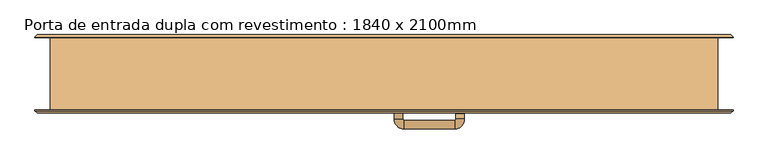
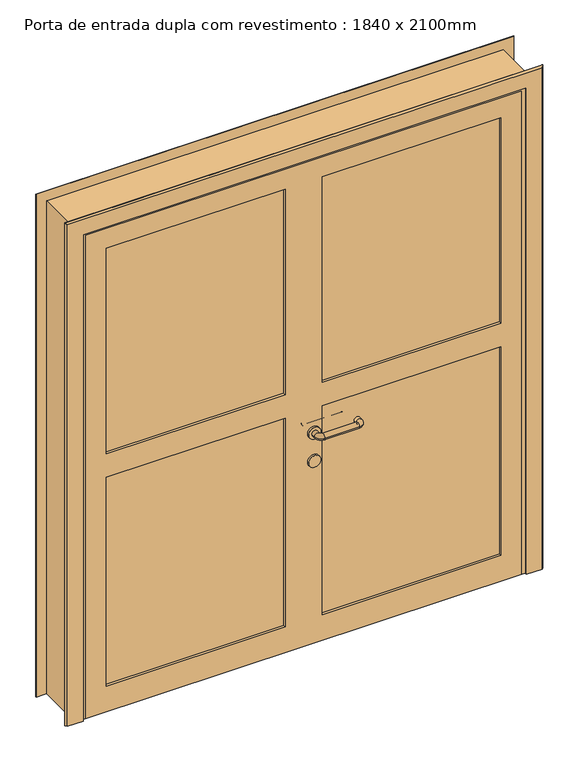
"""IFC4 building model written with IfcOpenShell, lengths in millimetres: door geometry, Porta de entrada dupla com revestimento : 1840 x 2100mm."""

import ifcopenshell
import ifcopenshell.guid

model = None  # the IFC model being written
_history = None  # IfcOwnerHistory: only IFC2X3 demands one
_inside = {}  # id of a spatial element -> (the spatial element, [elements in it])
_under = {}  # id of a project, library or spatial element -> (it, [spatial elements below it])
_declared = {}  # id of a project -> (the project, [libraries it declares])
_typed = {}  # id of a type object -> (the type object, [elements of that type])
_made_of = {}  # id of a material, layer set ... -> (it, [elements and type objects made of it])


def new_model(schema):
    """Start an empty IFC model of exactly this schema.

    Asked for "IFC4X3", IfcOpenShell would pick the latest addendum, in which some entities
    have other attributes; the version numbers below select the first issue.
    IFC2X3 requires an IfcOwnerHistory on every rooted entity: one is made here for all.
    """
    global model, _history
    if schema == "IFC4X3":
        model = ifcopenshell.file(schema_version=(4, 3, 0, 0))
    else:
        model = ifcopenshell.file(schema=schema)
    _inside.clear()
    _under.clear()
    _declared.clear()
    _typed.clear()
    _made_of.clear()
    _history = None
    if model.schema == "IFC2X3":
        org = make("IfcOrganization", Name="unknown")
        user = make(
            "IfcPersonAndOrganization",
            ThePerson=make("IfcPerson", FamilyName="unknown"),
            TheOrganization=org,
        )
        app = make(
            "IfcApplication",
            ApplicationDeveloper=org,
            Version="unknown",
            ApplicationFullName="unknown",
            ApplicationIdentifier="unknown",
        )
        _history = make(
            "IfcOwnerHistory",
            OwningUser=user,
            OwningApplication=app,
            ChangeAction="ADDED",
            CreationDate=0,
        )
    return model


def make(cls, **values):
    """One entity of the class cls with the attributes given. An attribute that is None is left unset."""
    return model.create_entity(
        cls, **{name: value for name, value in values.items() if value is not None}
    )


def rooted(cls, **values):
    """An entity with a GlobalId (a new one), such as an element, a storey or a relation."""
    return make(cls, GlobalId=ifcopenshell.guid.new(), OwnerHistory=_history, **values)


def si_unit(unit_type, name, prefix=None):
    """IfcSIUnit, for example si_unit("LENGTHUNIT", "METRE", prefix="MILLI")."""
    return make("IfcSIUnit", UnitType=unit_type, Prefix=prefix, Name=name)


def assignment(units):
    """IfcUnitAssignment: the units of a project."""
    return None if units is None else make("IfcUnitAssignment", Units=units)


def point(xyz):
    """IfcCartesianPoint."""
    return None if xyz is None else make("IfcCartesianPoint", Coordinates=xyz)


def direction(xyz):
    """IfcDirection."""
    return None if xyz is None else make("IfcDirection", DirectionRatios=xyz)


def frame(location, z_axis=None, x_axis=None):
    """IfcAxis2Placement3D, a coordinate frame: its origin and axes. An axis left out is left unset."""
    return make(
        "IfcAxis2Placement3D",
        Location=point(location),
        Axis=direction(z_axis),
        RefDirection=direction(x_axis),
    )


def frame_2d(location, x_axis=None):
    """IfcAxis2Placement2D, a coordinate frame in the plane: its origin and x axis."""
    return make(
        "IfcAxis2Placement2D", Location=point(location), RefDirection=direction(x_axis)
    )


def origin():
    """The frame at (0, 0, 0) with its axes left unset."""
    return frame((0.0, 0.0, 0.0))


def place(relative_to, where):
    """IfcLocalPlacement: puts the frame where relative to a parent placement (None: the world)."""
    return make(
        "IfcLocalPlacement", PlacementRelTo=relative_to, RelativePlacement=where
    )


def context(
    kind, dimensions, precision=None, world=None, true_north=None, identifier=None
):
    """IfcGeometricRepresentationContext, for example the 3D "Model" context."""
    return make(
        "IfcGeometricRepresentationContext",
        ContextIdentifier=identifier,
        ContextType=kind,
        CoordinateSpaceDimension=dimensions,
        Precision=precision,
        WorldCoordinateSystem=world,
        TrueNorth=true_north,
    )


def project(units=None, contexts=None):
    """IfcProject with its units and contexts."""
    return rooted(
        "IfcProject",
        Name="project",
        RepresentationContexts=contexts,
        UnitsInContext=assignment(units),
    )


def spatial(cls, under=None, at=None, **own):
    """A site, building, storey or space (cls), placed at a placement, below another one or the project."""
    s = rooted(cls, ObjectPlacement=at, **own)
    if under is not None:
        _under.setdefault(under.id(), (under, []))[1].append(s)
    return s


def polyline(points):
    """IfcPolyline through the points."""
    return make("IfcPolyline", Points=[point(p) for p in points])


def circle_curve(where, radius):
    """IfcCircle in the frame where."""
    return make("IfcCircle", Position=where, Radius=radius)


def ellipse_curve(where, semi_axis1, semi_axis2):
    """IfcEllipse in the frame where."""
    return make(
        "IfcEllipse", Position=where, SemiAxis1=semi_axis1, SemiAxis2=semi_axis2
    )


def trimmed(basis, trim1, trim2, sense, master):
    """IfcTrimmedCurve: the piece of a basis curve between two trims."""
    return make(
        "IfcTrimmedCurve",
        BasisCurve=basis,
        Trim1=trim1,
        Trim2=trim2,
        SenseAgreement=sense,
        MasterRepresentation=master,
    )


def segment(curve, same_sense, transition):
    """IfcCompositeCurveSegment."""
    return make(
        "IfcCompositeCurveSegment",
        Transition=transition,
        SameSense=same_sense,
        ParentCurve=curve,
    )


def composite_curve(segments, self_intersect=None):
    """IfcCompositeCurve: segments joined end to end."""
    return make("IfcCompositeCurve", Segments=segments, SelfIntersect=self_intersect)


def outline(outer, holes=None, kind="AREA"):
    """IfcArbitraryClosedProfileDef: a profile drawn as a closed curve; with holes, ...WithVoids."""
    if holes is None:
        return make("IfcArbitraryClosedProfileDef", ProfileType=kind, OuterCurve=outer)
    return make(
        "IfcArbitraryProfileDefWithVoids",
        ProfileType=kind,
        OuterCurve=outer,
        InnerCurves=holes,
    )


def extrude(swept, where, along, depth):
    """IfcExtrudedAreaSolid: the profile swept, set in the frame where, extruded along a direction by depth."""
    return make(
        "IfcExtrudedAreaSolid",
        SweptArea=swept,
        Position=where,
        ExtrudedDirection=direction(along),
        Depth=depth,
    )


def faces_of(points, faces, orient=None, outer=None):
    """IfcFace entities. A face is a list of loops; a loop is a list of indices into points, from 0.

    orient and outer hold one flag for each loop. By default every Orientation is true, the
    first loop of a face is its IfcFaceOuterBound and the others are IfcFaceBound.
    """
    made = []
    for i, loops in enumerate(faces):
        bounds = []
        for j, loop in enumerate(loops):
            is_outer = j == 0 if outer is None else outer[i][j]
            bounds.append(
                make(
                    "IfcFaceOuterBound" if is_outer else "IfcFaceBound",
                    Bound=make("IfcPolyLoop", Polygon=[points[k] for k in loop]),
                    Orientation=True if orient is None else orient[i][j],
                )
            )
        made.append(make("IfcFace", Bounds=bounds))
    return made


def faceted_brep(points, faces, orient=None, outer=None, voids=None):
    """IfcFacetedBrep: a solid bounded by flat faces; with voids (closed shells), ...WithVoids."""
    shared = [point(p) for p in points]
    hull = make("IfcClosedShell", CfsFaces=faces_of(shared, faces, orient, outer))
    if voids is None:
        return make("IfcFacetedBrep", Outer=hull)
    return make(
        "IfcFacetedBrepWithVoids",
        Outer=hull,
        Voids=[
            make(cls, CfsFaces=faces_of(shared, fs, o, b)) for cls, fs, o, b in voids
        ],
    )


def shape(context_of_items, identifier, shape_type, items):
    """IfcShapeRepresentation: the items that make up one representation, for example the "Body"."""
    return make(
        "IfcShapeRepresentation",
        ContextOfItems=context_of_items,
        RepresentationIdentifier=identifier,
        RepresentationType=shape_type,
        Items=items,
    )


def source(mapping_origin, context_of_items, identifier, shape_type, items):
    """IfcRepresentationMap: a shape defined once, which mapped items show again and again."""
    return make(
        "IfcRepresentationMap",
        MappingOrigin=mapping_origin,
        MappedRepresentation=shape(context_of_items, identifier, shape_type, items),
    )


def transform(
    local_origin,
    x_axis=None,
    y_axis=None,
    z_axis=None,
    scale=None,
    scale2=None,
    scale3=None,
    uniform=True,
):
    """IfcCartesianTransformationOperator3D, or its non-uniform kind. x_axis, y_axis, z_axis: its Axis1, 2, 3."""
    if uniform:
        return make(
            "IfcCartesianTransformationOperator3D",
            Axis1=direction(x_axis),
            Axis2=direction(y_axis),
            LocalOrigin=point(local_origin),
            Scale=scale,
            Axis3=direction(z_axis),
        )
    return make(
        "IfcCartesianTransformationOperator3DnonUniform",
        Axis1=direction(x_axis),
        Axis2=direction(y_axis),
        LocalOrigin=point(local_origin),
        Scale=scale,
        Axis3=direction(z_axis),
        Scale2=scale2,
        Scale3=scale3,
    )


def mapped(mapping_source, mapping_target):
    """IfcMappedItem: shows the shape of a source again, moved by a transform."""
    return make(
        "IfcMappedItem", MappingSource=mapping_source, MappingTarget=mapping_target
    )


def made_of(thing, what):
    """Note that an element or type object is made of a material, layer set ...; save() writes the relation."""
    if what is not None:
        _made_of.setdefault(what.id(), (what, []))[1].append(thing)
    return thing


def element(
    cls,
    number,
    at=None,
    inside=None,
    cuts=None,
    type_object=None,
    material=None,
    context=None,
    identifier="Body",
    shape_type=None,
    held_by="IfcProductDefinitionShape",
    body=None,
    shapes=None,
    **own,
):
    """One element of the class cls, such as IfcWall. Its Tag is "e" and its number.

    at: its placement. inside: the storey or other place that contains it. cuts: it is an
    opening in that element (IfcRelVoidsElement). A single representation is given by context,
    identifier, shape_type and body (its items); several are given by shapes. held_by: the class
    of the entity that holds the representations. save() writes the other relations.
    """
    e = rooted(cls, Tag="e%d" % number, ObjectPlacement=at, **own)
    if body is not None:
        shapes = [shape(context, identifier, shape_type, body)]
    if shapes is not None:
        e.Representation = make(held_by, Representations=shapes)
    if inside is not None:
        _inside.setdefault(inside.id(), (inside, []))[1].append(e)
    if cuts is not None:
        rooted(
            "IfcRelVoidsElement", RelatingBuildingElement=cuts, RelatedOpeningElement=e
        )
    if type_object is not None:
        _typed.setdefault(type_object.id(), (type_object, []))[1].append(e)
    return made_of(e, material)


def aggregate(whole, parts):
    """IfcRelAggregates: a whole, such as a stair, and the parts it consists of."""
    return rooted("IfcRelAggregates", RelatingObject=whole, RelatedObjects=parts)


def save(model, path):
    """Write the relations noted so far, then the file.

    IfcRelAggregates (storeys below a building ...), IfcRelContainedInSpatialStructure (elements
    in a storey), IfcRelDefinesByType, IfcRelAssociatesMaterial and IfcRelDeclares: one each for
    every whole, place, type object, material and project.
    """
    for whole, parts in _under.values():
        aggregate(whole, parts)
    for where, things in _inside.values():
        rooted(
            "IfcRelContainedInSpatialStructure",
            RelatedElements=things,
            RelatingStructure=where,
        )
    for kind, things in _typed.values():
        rooted("IfcRelDefinesByType", RelatedObjects=things, RelatingType=kind)
    for what, things in _made_of.values():
        rooted("IfcRelAssociatesMaterial", RelatedObjects=things, RelatingMaterial=what)
    for by, libraries in _declared.values():
        rooted("IfcRelDeclares", RelatingContext=by, RelatedDefinitions=libraries)
    model.write(path)


def plane_surface(at):
    """IfcPlane: the flat surface through the origin of the frame at, square to its z axis."""
    return make("IfcPlane", Position=at)


def cylinder_surface(at, radius):
    """IfcCylindricalSurface: all points at the distance radius from the z axis of the frame at."""
    return make("IfcCylindricalSurface", Position=at, Radius=radius)


def revolved_surface(curve, axis_point, axis_direction):
    """IfcSurfaceOfRevolution: the curve turned about the line through axis_point along axis_direction."""
    return make(
        "IfcSurfaceOfRevolution",
        SweptCurve=make("IfcArbitraryOpenProfileDef", ProfileType="CURVE", Curve=curve),
        AxisPosition=make("IfcAxis1Placement", Location=point(axis_point), Axis=direction(axis_direction)),
    )


def advanced_brep(points, edges, surfaces, faces):
    """IfcAdvancedBrep: a solid bounded by faces that lie on surfaces and meet in shared edges.

    An edge is (start, end): straight between two places in points (the first is 0);
    or (start, end, curve); or (start, end, curve, False) where it runs against its curve.
    A face is (place in surfaces, loops), or (place, loops, False) where it looks against
    its surface's normal. A loop lists edges by number (the first is 1), with a minus sign
    where the edge is run from its end to its start. The first loop is the outer one.
    """
    corners = [point(p) for p in points]
    vertices = [make("IfcVertexPoint", VertexGeometry=c) for c in corners]
    made = []
    for start, end, *more in edges:
        made.append(
            make(
                "IfcEdgeCurve",
                EdgeStart=vertices[start],
                EdgeEnd=vertices[end],
                EdgeGeometry=more[0] if more else make("IfcPolyline", Points=[corners[start], corners[end]]),
                SameSense=more[1] if len(more) > 1 else True,
            )
        )
    hull = []
    for where, loops, *sense in faces:
        bounds = []
        for j, loop in enumerate(loops):
            ring = [make("IfcOrientedEdge", EdgeElement=made[abs(k) - 1], Orientation=k > 0) for k in loop]
            bounds.append(
                make(
                    "IfcFaceOuterBound" if j == 0 else "IfcFaceBound",
                    Bound=make("IfcEdgeLoop", EdgeList=ring),
                    Orientation=True,
                )
            )
        hull.append(make("IfcAdvancedFace", Bounds=bounds, FaceSurface=surfaces[where], SameSense=sense[0] if sense else True))
    return make("IfcAdvancedBrep", Outer=make("IfcClosedShell", CfsFaces=hull))


def porta_de_entrada_dupla_com_revestimento_1840_x_2100mm_8bed4eb5(model_context):
    return source(origin(), model_context, "Body", "SolidModel", [
        advanced_brep(
        [(52.0, -57.0, 900.0), (28.0, -57.0, 900.0), (52.0, -40.0, 900.0), (28.0, -40.0, 900.0), (55.0, -13.0, 900.0), (55.0, -37.0, 900.0), (195.0, -37.0, 900.0), (195.0, -13.0, 900.0), (222.0, -40.0, 900.0), (198.0, -40.0, 900.0), (198.0, -55.0, 900.0), (222.0, -55.0, 900.0)],
        [
            (0, 1, circle_curve(frame((40.0, -57.0, 900.0), z_axis=(0.0, -1.0, 0.0), x_axis=(-1.0, 0.0, 0.0)), 12.0)),
            (1, 0, circle_curve(frame((40.0, -57.0, 900.0), z_axis=(0.0, -1.0, 0.0), x_axis=(-1.0, 0.0, 0.0)), 12.0)),
            (0, 2),
            (2, 3, circle_curve(frame((40.0, -40.0, 900.0), z_axis=(0.0, -1.0, 0.0), x_axis=(-1.0, 0.0, 0.0)), 12.0)),
            (3, 1),
            (3, 2, circle_curve(frame((40.0, -40.0, 900.0), z_axis=(0.0, -1.0, 0.0), x_axis=(-1.0, 0.0, 0.0)), 12.0)),
            (4, 3, circle_curve(frame((55.0, -40.0, 900.0), z_axis=(0.0, 0.0, 1.0), x_axis=(-1.0, 0.0, 0.0)), 27.0)),
            (2, 5, circle_curve(frame((55.0, -40.0, 900.0), z_axis=(0.0, 0.0, -1.0), x_axis=(-1.0, 0.0, 0.0)), 3.0)),
            (5, 4, circle_curve(frame((55.0, -25.0, 900.0), z_axis=(-1.0, 0.0, 0.0), x_axis=(0.0, 1.0, 0.0)), 12.0)),
            (4, 5, circle_curve(frame((55.0, -25.0, 900.0), z_axis=(-1.0, 0.0, 0.0), x_axis=(0.0, 1.0, 0.0)), 12.0)),
            (5, 6),
            (6, 7, circle_curve(frame((195.0, -25.0, 900.0), z_axis=(-1.0, 0.0, 0.0), x_axis=(0.0, 1.0, 0.0)), 12.0)),
            (7, 4),
            (7, 6, circle_curve(frame((195.0, -25.0, 900.0), z_axis=(-1.0, 0.0, 0.0), x_axis=(0.0, 1.0, 0.0)), 12.0)),
            (8, 7, circle_curve(frame((195.0, -40.0, 900.0), z_axis=(0.0, 0.0, 1.0), x_axis=(0.0, 1.0, 0.0)), 27.0)),
            (6, 9, circle_curve(frame((195.0, -40.0, 900.0), z_axis=(0.0, 0.0, -1.0), x_axis=(0.0, 1.0, 0.0)), 3.0)),
            (9, 8, circle_curve(frame((210.0, -40.0, 900.0), z_axis=(0.0, 1.0, 0.0), x_axis=(1.0, 0.0, 0.0)), 12.0)),
            (8, 9, circle_curve(frame((210.0, -40.0, 900.0), z_axis=(0.0, 1.0, 0.0), x_axis=(1.0, 0.0, 0.0)), 12.0)),
            (10, 11, circle_curve(frame((210.0, -55.0, 900.0), z_axis=(0.0, -1.0, 0.0), x_axis=(1.0, 0.0, 0.0)), 12.0)),
            (11, 10, circle_curve(frame((210.0, -55.0, 900.0), z_axis=(0.0, -1.0, 0.0), x_axis=(1.0, 0.0, 0.0)), 12.0)),
            (9, 10),
            (11, 8),
        ],
        [
            plane_surface(frame((-802.0, -57.0, 1730.0), z_axis=(0.0, -1.0, 0.0), x_axis=(0.0, 0.0, 1.0))),
            cylinder_surface(frame((40.0, -57.0, 900.0), z_axis=(0.0, -1.0, 0.0), x_axis=(-1.0, 0.0, 0.0)), 12.0),
            revolved_surface(trimmed(ellipse_curve(frame((40.0, -40.0, 900.0), z_axis=(0.0, -1.0, 0.0), x_axis=(-1.0, 0.0, 0.0)), 12.0, 12.0), [point((52.0, -40.0, 900.0))], [point((28.0, -40.0, 900.0))], True, "CARTESIAN"), (55.0, -40.0, 1730.0), (0.0, 0.0, -1.0)),
            revolved_surface(trimmed(ellipse_curve(frame((40.0, -40.0, 900.0), z_axis=(0.0, -1.0, 0.0), x_axis=(-1.0, 0.0, 0.0)), 12.0, 12.0), [point((28.0, -40.0, 900.0))], [point((52.0, -40.0, 900.0))], True, "CARTESIAN"), (55.0, -40.0, 1730.0), (0.0, 0.0, -1.0)),
            cylinder_surface(frame((55.0, -25.0, 900.0), z_axis=(-1.0, 0.0, 0.0), x_axis=(0.0, 1.0, 0.0)), 12.0),
            revolved_surface(trimmed(ellipse_curve(frame((195.0, -25.0, 900.0), z_axis=(-1.0, 0.0, 0.0), x_axis=(0.0, 1.0, 0.0)), 12.0, 12.0), [point((195.0, -37.0, 900.0))], [point((195.0, -13.0, 900.0))], True, "CARTESIAN"), (195.0, -40.0, 1730.0), (0.0, 0.0, -1.0)),
            revolved_surface(trimmed(ellipse_curve(frame((195.0, -25.0, 900.0), z_axis=(-1.0, 0.0, 0.0), x_axis=(0.0, 1.0, 0.0)), 12.0, 12.0), [point((195.0, -13.0, 900.0))], [point((195.0, -37.0, 900.0))], True, "CARTESIAN"), (195.0, -40.0, 1730.0), (0.0, 0.0, -1.0)),
            plane_surface(frame((-632.0, -55.0, 1730.0), z_axis=(0.0, -1.0, 0.0), x_axis=(0.0, 0.0, -1.0))),
            cylinder_surface(frame((210.0, -40.0, 900.0), z_axis=(0.0, 1.0, 0.0), x_axis=(1.0, 0.0, 0.0)), 12.0),
        ],
        [
            (0, [[1, 2]]),
            (1, [[-1, 3, 4, 5]]),
            (1, [[-2, -5, 6, -3]]),
            (2, [[7, -4, 8, 9]]),
            (3, [[-8, -6, -7, 10]]),
            (4, [[-9, 11, 12, 13]]),
            (4, [[-10, -13, 14, -11]]),
            (5, [[15, -12, 16, 17]]),
            (6, [[-16, -14, -15, 18]]),
            (7, [[19, 20]]),
            (8, [[-17, 21, -20, 22]]),
            (8, [[-18, -22, -19, -21]]),
        ],
    ),
        extrude(outline(composite_curve([segment(trimmed(circle_curve(frame_2d((780.0, 40.0)), 25.0), [point((780.0, 15.0))], [point((780.0, 65.0))], False, "CARTESIAN"), True, "CONTINUOUS"), segment(trimmed(circle_curve(frame_2d((780.0, 40.0)), 25.0), [point((780.0, 65.0))], [point((780.0, 15.0))], False, "CARTESIAN"), True, "CONTINUOUS")], self_intersect=False)), frame((0.0, -65.0, 0.0), z_axis=(0.0, 1.0, 0.0), x_axis=(0.0, 0.0, 1.0)), (0.0, 0.0, 1.0), 8.0),
        extrude(outline(composite_curve([segment(trimmed(circle_curve(frame_2d((900.0, 40.0)), 25.0), [point((900.0, 15.0))], [point((900.0, 65.0))], False, "CARTESIAN"), True, "CONTINUOUS"), segment(trimmed(circle_curve(frame_2d((900.0, 40.0)), 25.0), [point((900.0, 65.0))], [point((900.0, 15.0))], False, "CARTESIAN"), True, "CONTINUOUS")], self_intersect=False)), frame((0.0, -65.0, 0.0), z_axis=(0.0, 1.0, 0.0), x_axis=(0.0, 0.0, 1.0)), (0.0, 0.0, 1.0), 8.0),
        advanced_brep(
        [(28.0, -108.0, 900.0), (52.0, -108.0, 900.0), (28.0, -125.0, 900.0), (52.0, -125.0, 900.0), (55.0, -128.0, 900.0), (55.0, -152.0, 900.0), (195.0, -152.0, 900.0), (195.0, -128.0, 900.0), (198.0, -125.0, 900.0), (222.0, -125.0, 900.0), (222.0, -110.0, 900.0), (198.0, -110.0, 900.0)],
        [
            (0, 1, circle_curve(frame((40.0, -108.0, 900.0), z_axis=(0.0, 1.0, 0.0), x_axis=(1.0, 0.0, 0.0)), 12.0)),
            (1, 0, circle_curve(frame((40.0, -108.0, 900.0), z_axis=(0.0, 1.0, 0.0), x_axis=(1.0, 0.0, 0.0)), 12.0)),
            (0, 2),
            (2, 3, circle_curve(frame((40.0, -125.0, 900.0), z_axis=(0.0, 1.0, 0.0), x_axis=(1.0, 0.0, 0.0)), 12.0)),
            (3, 1),
            (3, 2, circle_curve(frame((40.0, -125.0, 900.0), z_axis=(0.0, 1.0, 0.0), x_axis=(1.0, 0.0, 0.0)), 12.0)),
            (4, 3, circle_curve(frame((55.0, -125.0, 900.0), z_axis=(0.0, 0.0, -1.0), x_axis=(-1.0, 0.0, 0.0)), 3.0)),
            (2, 5, circle_curve(frame((55.0, -125.0, 900.0), z_axis=(0.0, 0.0, 1.0), x_axis=(-1.0, 0.0, 0.0)), 27.0)),
            (5, 4, circle_curve(frame((55.0, -140.0, 900.0), z_axis=(-1.0, 0.0, 0.0), x_axis=(0.0, 1.0, 0.0)), 12.0)),
            (4, 5, circle_curve(frame((55.0, -140.0, 900.0), z_axis=(-1.0, 0.0, 0.0), x_axis=(0.0, 1.0, 0.0)), 12.0)),
            (5, 6),
            (6, 7, circle_curve(frame((195.0, -140.0, 900.0), z_axis=(-1.0, 0.0, 0.0), x_axis=(0.0, 1.0, 0.0)), 12.0)),
            (7, 4),
            (7, 6, circle_curve(frame((195.0, -140.0, 900.0), z_axis=(-1.0, 0.0, 0.0), x_axis=(0.0, 1.0, 0.0)), 12.0)),
            (8, 7, circle_curve(frame((195.0, -125.0, 900.0), z_axis=(0.0, 0.0, -1.0), x_axis=(0.0, -1.0, 0.0)), 3.0)),
            (6, 9, circle_curve(frame((195.0, -125.0, 900.0), z_axis=(0.0, 0.0, 1.0), x_axis=(0.0, -1.0, 0.0)), 27.0)),
            (9, 8, circle_curve(frame((210.0, -125.0, 900.0), z_axis=(0.0, -1.0, 0.0), x_axis=(-1.0, 0.0, 0.0)), 12.0)),
            (8, 9, circle_curve(frame((210.0, -125.0, 900.0), z_axis=(0.0, -1.0, 0.0), x_axis=(-1.0, 0.0, 0.0)), 12.0)),
            (10, 11, circle_curve(frame((210.0, -110.0, 900.0), z_axis=(0.0, 1.0, 0.0), x_axis=(-1.0, 0.0, 0.0)), 12.0)),
            (11, 10, circle_curve(frame((210.0, -110.0, 900.0), z_axis=(0.0, 1.0, 0.0), x_axis=(-1.0, 0.0, 0.0)), 12.0)),
            (9, 10),
            (11, 8),
        ],
        [
            plane_surface(frame((-802.0, -108.0, 1730.0), z_axis=(0.0, 1.0, 0.0), x_axis=(0.0, 0.0, -1.0))),
            cylinder_surface(frame((40.0, -108.0, 900.0), z_axis=(0.0, 1.0, 0.0), x_axis=(1.0, 0.0, 0.0)), 12.0),
            revolved_surface(trimmed(ellipse_curve(frame((40.0, -125.0, 900.0), z_axis=(0.0, 1.0, 0.0), x_axis=(1.0, 0.0, 0.0)), 12.0, 12.0), [point((28.0, -125.0, 900.0))], [point((52.0, -125.0, 900.0))], True, "CARTESIAN"), (55.0, -125.0, 1730.0), (0.0, 0.0, 1.0)),
            revolved_surface(trimmed(ellipse_curve(frame((40.0, -125.0, 900.0), z_axis=(0.0, 1.0, 0.0), x_axis=(1.0, 0.0, 0.0)), 12.0, 12.0), [point((52.0, -125.0, 900.0))], [point((28.0, -125.0, 900.0))], True, "CARTESIAN"), (55.0, -125.0, 1730.0), (0.0, 0.0, 1.0)),
            cylinder_surface(frame((55.0, -140.0, 900.0), z_axis=(-1.0, 0.0, 0.0), x_axis=(0.0, 1.0, 0.0)), 12.0),
            revolved_surface(trimmed(ellipse_curve(frame((195.0, -140.0, 900.0), z_axis=(-1.0, 0.0, 0.0), x_axis=(0.0, 1.0, 0.0)), 12.0, 12.0), [point((195.0, -152.0, 900.0))], [point((195.0, -128.0, 900.0))], True, "CARTESIAN"), (195.0, -125.0, 1730.0), (0.0, 0.0, 1.0)),
            revolved_surface(trimmed(ellipse_curve(frame((195.0, -140.0, 900.0), z_axis=(-1.0, 0.0, 0.0), x_axis=(0.0, 1.0, 0.0)), 12.0, 12.0), [point((195.0, -128.0, 900.0))], [point((195.0, -152.0, 900.0))], True, "CARTESIAN"), (195.0, -125.0, 1730.0), (0.0, 0.0, 1.0)),
            plane_surface(frame((-632.0, -110.0, 1730.0), z_axis=(0.0, 1.0, 0.0), x_axis=(0.0, 0.0, 1.0))),
            cylinder_surface(frame((210.0, -125.0, 900.0), z_axis=(0.0, -1.0, 0.0), x_axis=(-1.0, 0.0, 0.0)), 12.0),
        ],
        [
            (0, [[1, 2]]),
            (1, [[-1, 3, 4, 5]]),
            (1, [[-2, -5, 6, -3]]),
            (2, [[7, -4, 8, 9]]),
            (3, [[-8, -6, -7, 10]]),
            (4, [[-9, 11, 12, 13]]),
            (4, [[-10, -13, 14, -11]]),
            (5, [[15, -12, 16, 17]]),
            (6, [[-16, -14, -15, 18]]),
            (7, [[19, 20]]),
            (8, [[-17, 21, -20, 22]]),
            (8, [[-18, -22, -19, -21]]),
        ],
    ),
        extrude(outline(composite_curve([segment(trimmed(circle_curve(frame_2d((780.0, 40.0)), 25.0), [point((780.0, 15.0))], [point((780.0, 65.0))], False, "CARTESIAN"), True, "CONTINUOUS"), segment(trimmed(circle_curve(frame_2d((780.0, 40.0)), 25.0), [point((780.0, 65.0))], [point((780.0, 15.0))], False, "CARTESIAN"), True, "CONTINUOUS")], self_intersect=False)), frame((0.0, -108.0, 0.0), z_axis=(0.0, 1.0, 0.0), x_axis=(0.0, 0.0, 1.0)), (0.0, 0.0, 1.0), 8.0),
        extrude(outline(composite_curve([segment(trimmed(circle_curve(frame_2d((900.0, 40.0)), 25.0), [point((900.0, 15.0))], [point((900.0, 65.0))], False, "CARTESIAN"), True, "CONTINUOUS"), segment(trimmed(circle_curve(frame_2d((900.0, 40.0)), 25.0), [point((900.0, 65.0))], [point((900.0, 15.0))], False, "CARTESIAN"), True, "CONTINUOUS")], self_intersect=False)), frame((0.0, -108.0, 0.0), z_axis=(0.0, 1.0, 0.0), x_axis=(0.0, 0.0, 1.0)), (0.0, 0.0, 1.0), 8.0),
        extrude(outline(polyline([(-835.0, -75.5), (835.0, -75.5), (835.0, -89.5), (-835.0, -89.5), (-835.0, -75.5)])), frame((0.0, 0.0, 70.0), z_axis=(0.0, 0.0, 1.0), x_axis=(1.0, 0.0, 0.0)), (0.0, 0.0, 1.0), 970.0),
        extrude(outline(polyline([(-835.0, -75.5), (835.0, -75.5), (835.0, -89.5), (-835.0, -89.5), (-835.0, -75.5)])), frame((0.0, 0.0, 1060.0), z_axis=(0.0, 0.0, 1.0), x_axis=(1.0, 0.0, 0.0)), (0.0, 0.0, 1.0), 955.0),
        extrude(outline(polyline([(-835.0, -75.5), (835.0, -75.5), (835.0, -89.5), (-835.0, -89.5), (-835.0, -75.5)])), frame((0.0, 0.0, 70.0), z_axis=(0.0, 0.0, 1.0), x_axis=(1.0, 0.0, 0.0)), (0.0, 0.0, 1.0), 970.0),
        extrude(outline(polyline([(-835.0, -75.5), (835.0, -75.5), (835.0, -89.5), (-835.0, -89.5), (-835.0, -75.5)])), frame((0.0, 0.0, 1060.0), z_axis=(0.0, 0.0, 1.0), x_axis=(1.0, 0.0, 0.0)), (0.0, 0.0, 1.0), 955.0),
        faceted_brep([(-920.0, 100.0, 0.0), (-870.0, 100.0, 0.0), (-870.0, -62.0, 0.0), (-880.0, -62.0, 0.0), (-880.0, -100.0, 0.0), (-920.0, -100.0, 0.0), (-920.0, 100.0, 2100.0), (920.0, 100.0, 2100.0), (920.0, 100.0, 0.0), (870.0, 100.0, 0.0), (870.0, 100.0, 2050.0), (-870.0, 100.0, 2050.0), (-870.0, -62.0, 2050.0), (870.0, -62.0, 2050.0), (870.0, -62.0, 0.0), (880.0, -62.0, 0.0), (880.0, -62.0, 2060.0), (-880.0, -62.0, 2060.0), (-880.0, -100.0, 2060.0), (880.0, -100.0, 2060.0), (880.0, -100.0, 0.0), (920.0, -100.0, 0.0), (920.0, -100.0, 2100.0), (-920.0, -100.0, 2100.0)], [[[0, 1, 2, 3, 4, 5]], [[1, 0, 6, 7, 8, 9, 10, 11]], [[2, 1, 11, 12]], [[3, 2, 12, 13, 14, 15, 16, 17]], [[4, 3, 17, 18]], [[5, 4, 18, 19, 20, 21, 22, 23]], [[0, 5, 23, 6]], [[7, 22, 21, 8]], [[8, 21, 20, 15, 14, 9]], [[13, 10, 9, 14]], [[19, 16, 15, 20]], [[12, 11, 10, 13]], [[18, 17, 16, 19]], [[6, 23, 22, 7]]]),
        faceted_brep([(963.0, -102.0, 0.0), (957.0, -108.0, 0.0), (893.0, -108.0, 0.0), (893.0, -100.0, 0.0), (963.0, -100.0, 0.0), (963.0, -102.0, 2143.0), (957.0, -108.0, 2137.0), (-957.0, -108.0, 2137.0), (-957.0, -108.0, 0.0), (-893.0, -108.0, 0.0), (-893.0, -108.0, 2073.0), (893.0, -108.0, 2073.0), (893.0, -100.0, 2073.0), (-893.0, -100.0, 2073.0), (-893.0, -100.0, 0.0), (-963.0, -100.0, 0.0), (-963.0, -100.0, 2143.0), (963.0, -100.0, 2143.0), (-963.0, -102.0, 2143.0), (-963.0, -102.0, 0.0)], [[[0, 1, 2, 3, 4]], [[1, 0, 5, 6]], [[2, 1, 6, 7, 8, 9, 10, 11]], [[3, 2, 11, 12]], [[4, 3, 12, 13, 14, 15, 16, 17]], [[0, 4, 17, 5]], [[7, 18, 19, 8]], [[19, 15, 14, 9, 8]], [[13, 10, 9, 14]], [[18, 16, 15, 19]], [[6, 5, 18, 7]], [[12, 11, 10, 13]], [[5, 17, 16, 18]]]),
        faceted_brep([(-963.0, 102.0, 0.0), (-957.0, 108.0, 0.0), (-893.0, 108.0, 0.0), (-893.0, 100.0, 0.0), (-963.0, 100.0, 0.0), (-963.0, 102.0, 2143.0), (-957.0, 108.0, 2137.0), (957.0, 108.0, 2137.0), (957.0, 108.0, 0.0), (893.0, 108.0, 0.0), (893.0, 108.0, 2073.0), (-893.0, 108.0, 2073.0), (-893.0, 100.0, 2073.0), (893.0, 100.0, 2073.0), (893.0, 100.0, 0.0), (963.0, 100.0, 0.0), (963.0, 100.0, 2143.0), (-963.0, 100.0, 2143.0), (963.0, 102.0, 2143.0), (963.0, 102.0, 0.0)], [[[0, 1, 2, 3, 4]], [[1, 0, 5, 6]], [[2, 1, 6, 7, 8, 9, 10, 11]], [[3, 2, 11, 12]], [[4, 3, 12, 13, 14, 15, 16, 17]], [[0, 4, 17, 5]], [[7, 18, 19, 8]], [[19, 15, 14, 9, 8]], [[13, 10, 9, 14]], [[18, 16, 15, 19]], [[6, 5, 18, 7]], [[12, 11, 10, 13]], [[5, 17, 16, 18]]]),
        extrude(outline(polyline([(2060.0, -880.0), (0.0, -880.0), (0.0, 880.0), (2060.0, 880.0), (2060.0, -880.0)]), holes=[polyline([(1975.0, 75.0), (1975.0, 795.0), (1100.0, 795.0), (1100.0, 75.0), (1975.0, 75.0)]), polyline([(1100.0, -795.0), (1975.0, -795.0), (1975.0, -75.0), (1100.0, -75.0), (1100.0, -795.0)]), polyline([(1000.0, 795.0), (110.0, 795.0), (110.0, 75.0), (1000.0, 75.0), (1000.0, 795.0)]), polyline([(110.0, -75.0), (110.0, -795.0), (1000.0, -795.0), (1000.0, -75.0), (110.0, -75.0)])]), frame((0.0, -100.0, 0.0), z_axis=(0.0, 1.0, 0.0), x_axis=(0.0, 0.0, 1.0)), (0.0, 0.0, 1.0), 35.0),
    ])


if __name__ == "__main__":
    model = new_model("IFC4")
    model_context = context("Model", 3, world=origin())
    ifc_project = project(units=[si_unit("LENGTHUNIT", "METRE", prefix="MILLI")], contexts=[model_context])
    site = spatial("IfcSite", under=ifc_project)
    building = spatial("IfcBuilding", under=site)
    placement = place(None, origin())
    porta_de_entrada_dupla_com_revestimento_1840_x_2100mm_shape = porta_de_entrada_dupla_com_revestimento_1840_x_2100mm_8bed4eb5(model_context)
    element("IfcDoor", 1, ObjectType="Porta de entrada dupla com revestimento : 1840 x 2100mm", at=placement, inside=building, context=model_context, shape_type="MappedRepresentation", body=[
        mapped(porta_de_entrada_dupla_com_revestimento_1840_x_2100mm_shape, transform((0.0, 0.0, 0.0), x_axis=(1.0, 0.0, 0.0), y_axis=(0.0, 1.0, 0.0), z_axis=(0.0, 0.0, 1.0))),
    ])
    save(model, "model.ifc")

# Revit data of these elements
# Type "Porta de entrada dupla com revestimento : 1840 x 2100mm"
#   Type Mark = "46"
#   Construction Type Id = "MDOOR"
#   Analytic Construction = "Metal"
#   W2 = 0.92 m
#   W1 = 1.76 m
#   Largura da apara = 0.07 m
#   Espessura da apara = 0.008 m
#   Thickness = 0.035 m
#   Rough Width = 1.84 m
#   Rough Height = 2.10 m
#   Largura da moldura do painel = 0.075 m
#   Heat Transfer Coefficient (U) = 3.7021 W/(m²·K)
#   Largura da estrutura = 0.05 m
#   Height = 2.10 m
#   Width = 1.84 m
#   Define Thermal Properties by = 1
#   Function = 1
#   Material da apara = none
#   Material do painel = none
#   Material do puxador = none
#   Vidro = none
#   Material da moldura = none
#   Visual Light Transmittance = 0
#   Solar Heat Gain Coefficient = 0
#   Wall Closure = (empty or 0)
# Element 1 (IfcDoor, "Porta de entrada dupla com revestimento : 1840 x 2100mm")
#   Materials on its faces: "Vidro"
# Materials
#   "Vidro": class "Vidro", colour RGB 0 128 192, transparency 0.9, Description = "Vidro de sílica", Cost = 0
